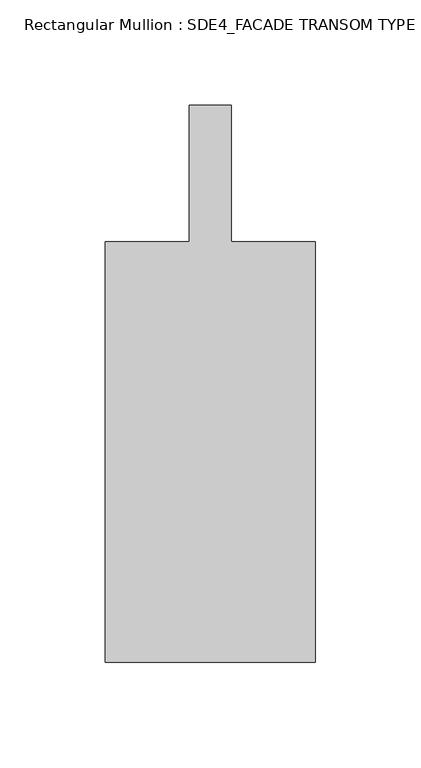
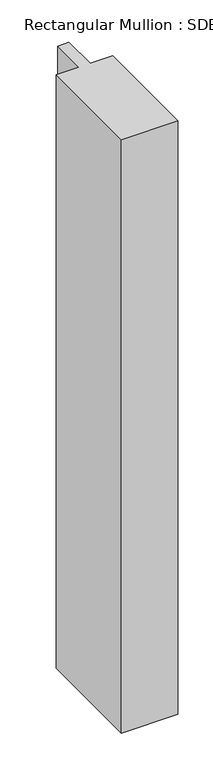
"""IFC4 building model written with IfcOpenShell, lengths in millimetres: member geometry, Rectangular Mullion : SDE4_FACADE TRANSOM TYPE 2."""

from ifc_helpers import new_model, si_unit, frame, origin, place, context, project, spatial, polyline, outline, extrude, source, transform, mapped, element, save


def rectangular_mullion_sde4_facade_transom_type_2_e58d2e59(model_context):
    return source(origin(), model_context, "Body", "SweptSolid", [
        extrude(outline(polyline([(50.0, -132.5), (-50.0, -132.5), (-50.0, 67.5), (-10.0, 67.5), (-10.0, 132.5), (10.0, 132.5), (10.0, 67.5), (50.0, 67.5), (50.0, -132.5)])), frame((0.0, 0.0, -1110.0), z_axis=(0.0, 0.0, 1.0), x_axis=(1.0, 0.0, 0.0)), (0.0, 0.0, 1.0), 1110.0),
    ])


if __name__ == "__main__":
    model = new_model("IFC4")
    model_context = context("Model", 3, world=origin())
    ifc_project = project(units=[si_unit("LENGTHUNIT", "METRE", prefix="MILLI")], contexts=[model_context])
    site = spatial("IfcSite", under=ifc_project)
    building = spatial("IfcBuilding", under=site)
    placement = place(None, origin())
    rectangular_mullion_sde4_facade_transom_type_2_shape = rectangular_mullion_sde4_facade_transom_type_2_e58d2e59(model_context)
    element("IfcMember", 1, ObjectType="Rectangular Mullion : SDE4_FACADE TRANSOM TYPE 2", at=placement, inside=building, context=model_context, shape_type="MappedRepresentation", body=[
        mapped(rectangular_mullion_sde4_facade_transom_type_2_shape, transform((0.0, 0.0, 0.0), x_axis=(1.0, 0.0, 0.0), y_axis=(0.0, 1.0, 0.0), z_axis=(0.0, 0.0, 1.0))),
    ])
    save(model, "model.ifc")

# Revit data of these elements
# Type "Rectangular Mullion : SDE4_FACADE TRANSOM TYPE 2"
#   built-in parameter 1007322 = 0.869423 (stored number, unit not read)
#   built-in parameter 1007321 = 0.164042 (stored number, unit not read)
#   built-in parameter 1007320 = 0.164042 (stored number, unit not read)
